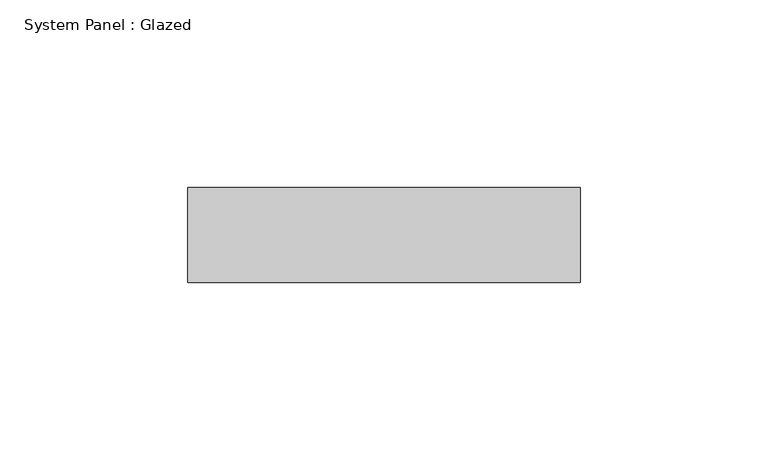
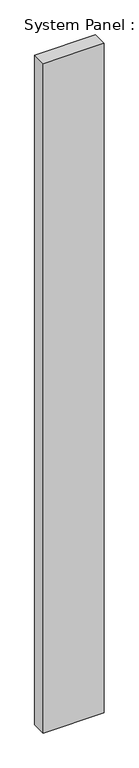
"""IFC4 building model written with IfcOpenShell, lengths in millimetres: plate geometry, System Panel : Glazed."""

import ifcopenshell
import ifcopenshell.guid

model = None  # the IFC model being written
_history = None  # IfcOwnerHistory: only IFC2X3 demands one
_inside = {}  # id of a spatial element -> (the spatial element, [elements in it])
_under = {}  # id of a project, library or spatial element -> (it, [spatial elements below it])
_declared = {}  # id of a project -> (the project, [libraries it declares])
_typed = {}  # id of a type object -> (the type object, [elements of that type])
_made_of = {}  # id of a material, layer set ... -> (it, [elements and type objects made of it])


def new_model(schema):
    """Start an empty IFC model of exactly this schema.

    Asked for "IFC4X3", IfcOpenShell would pick the latest addendum, in which some entities
    have other attributes; the version numbers below select the first issue.
    IFC2X3 requires an IfcOwnerHistory on every rooted entity: one is made here for all.
    """
    global model, _history
    if schema == "IFC4X3":
        model = ifcopenshell.file(schema_version=(4, 3, 0, 0))
    else:
        model = ifcopenshell.file(schema=schema)
    _inside.clear()
    _under.clear()
    _declared.clear()
    _typed.clear()
    _made_of.clear()
    _history = None
    if model.schema == "IFC2X3":
        org = make("IfcOrganization", Name="unknown")
        user = make(
            "IfcPersonAndOrganization",
            ThePerson=make("IfcPerson", FamilyName="unknown"),
            TheOrganization=org,
        )
        app = make(
            "IfcApplication",
            ApplicationDeveloper=org,
            Version="unknown",
            ApplicationFullName="unknown",
            ApplicationIdentifier="unknown",
        )
        _history = make(
            "IfcOwnerHistory",
            OwningUser=user,
            OwningApplication=app,
            ChangeAction="ADDED",
            CreationDate=0,
        )
    return model


def make(cls, **values):
    """One entity of the class cls with the attributes given. An attribute that is None is left unset."""
    return model.create_entity(
        cls, **{name: value for name, value in values.items() if value is not None}
    )


def rooted(cls, **values):
    """An entity with a GlobalId (a new one), such as an element, a storey or a relation."""
    return make(cls, GlobalId=ifcopenshell.guid.new(), OwnerHistory=_history, **values)


def si_unit(unit_type, name, prefix=None):
    """IfcSIUnit, for example si_unit("LENGTHUNIT", "METRE", prefix="MILLI")."""
    return make("IfcSIUnit", UnitType=unit_type, Prefix=prefix, Name=name)


def assignment(units):
    """IfcUnitAssignment: the units of a project."""
    return None if units is None else make("IfcUnitAssignment", Units=units)


def point(xyz):
    """IfcCartesianPoint."""
    return None if xyz is None else make("IfcCartesianPoint", Coordinates=xyz)


def direction(xyz):
    """IfcDirection."""
    return None if xyz is None else make("IfcDirection", DirectionRatios=xyz)


def frame(location, z_axis=None, x_axis=None):
    """IfcAxis2Placement3D, a coordinate frame: its origin and axes. An axis left out is left unset."""
    return make(
        "IfcAxis2Placement3D",
        Location=point(location),
        Axis=direction(z_axis),
        RefDirection=direction(x_axis),
    )


def origin():
    """The frame at (0, 0, 0) with its axes left unset."""
    return frame((0.0, 0.0, 0.0))


def origin_with_axes():
    """The frame at (0, 0, 0) with the z axis (0, 0, 1) and the x axis (1, 0, 0) written out."""
    return frame((0.0, 0.0, 0.0), z_axis=(0.0, 0.0, 1.0), x_axis=(1.0, 0.0, 0.0))


def place(relative_to, where):
    """IfcLocalPlacement: puts the frame where relative to a parent placement (None: the world)."""
    return make(
        "IfcLocalPlacement", PlacementRelTo=relative_to, RelativePlacement=where
    )


def context(
    kind, dimensions, precision=None, world=None, true_north=None, identifier=None
):
    """IfcGeometricRepresentationContext, for example the 3D "Model" context."""
    return make(
        "IfcGeometricRepresentationContext",
        ContextIdentifier=identifier,
        ContextType=kind,
        CoordinateSpaceDimension=dimensions,
        Precision=precision,
        WorldCoordinateSystem=world,
        TrueNorth=true_north,
    )


def project(units=None, contexts=None):
    """IfcProject with its units and contexts."""
    return rooted(
        "IfcProject",
        Name="project",
        RepresentationContexts=contexts,
        UnitsInContext=assignment(units),
    )


def spatial(cls, under=None, at=None, **own):
    """A site, building, storey or space (cls), placed at a placement, below another one or the project."""
    s = rooted(cls, ObjectPlacement=at, **own)
    if under is not None:
        _under.setdefault(under.id(), (under, []))[1].append(s)
    return s


def polyline(points):
    """IfcPolyline through the points."""
    return make("IfcPolyline", Points=[point(p) for p in points])


def outline(outer, holes=None, kind="AREA"):
    """IfcArbitraryClosedProfileDef: a profile drawn as a closed curve; with holes, ...WithVoids."""
    if holes is None:
        return make("IfcArbitraryClosedProfileDef", ProfileType=kind, OuterCurve=outer)
    return make(
        "IfcArbitraryProfileDefWithVoids",
        ProfileType=kind,
        OuterCurve=outer,
        InnerCurves=holes,
    )


def extrude(swept, where, along, depth):
    """IfcExtrudedAreaSolid: the profile swept, set in the frame where, extruded along a direction by depth."""
    return make(
        "IfcExtrudedAreaSolid",
        SweptArea=swept,
        Position=where,
        ExtrudedDirection=direction(along),
        Depth=depth,
    )


def shape(context_of_items, identifier, shape_type, items):
    """IfcShapeRepresentation: the items that make up one representation, for example the "Body"."""
    return make(
        "IfcShapeRepresentation",
        ContextOfItems=context_of_items,
        RepresentationIdentifier=identifier,
        RepresentationType=shape_type,
        Items=items,
    )


def source(mapping_origin, context_of_items, identifier, shape_type, items):
    """IfcRepresentationMap: a shape defined once, which mapped items show again and again."""
    return make(
        "IfcRepresentationMap",
        MappingOrigin=mapping_origin,
        MappedRepresentation=shape(context_of_items, identifier, shape_type, items),
    )


def transform(
    local_origin,
    x_axis=None,
    y_axis=None,
    z_axis=None,
    scale=None,
    scale2=None,
    scale3=None,
    uniform=True,
):
    """IfcCartesianTransformationOperator3D, or its non-uniform kind. x_axis, y_axis, z_axis: its Axis1, 2, 3."""
    if uniform:
        return make(
            "IfcCartesianTransformationOperator3D",
            Axis1=direction(x_axis),
            Axis2=direction(y_axis),
            LocalOrigin=point(local_origin),
            Scale=scale,
            Axis3=direction(z_axis),
        )
    return make(
        "IfcCartesianTransformationOperator3DnonUniform",
        Axis1=direction(x_axis),
        Axis2=direction(y_axis),
        LocalOrigin=point(local_origin),
        Scale=scale,
        Axis3=direction(z_axis),
        Scale2=scale2,
        Scale3=scale3,
    )


def mapped(mapping_source, mapping_target):
    """IfcMappedItem: shows the shape of a source again, moved by a transform."""
    return make(
        "IfcMappedItem", MappingSource=mapping_source, MappingTarget=mapping_target
    )


def made_of(thing, what):
    """Note that an element or type object is made of a material, layer set ...; save() writes the relation."""
    if what is not None:
        _made_of.setdefault(what.id(), (what, []))[1].append(thing)
    return thing


def element(
    cls,
    number,
    at=None,
    inside=None,
    cuts=None,
    type_object=None,
    material=None,
    context=None,
    identifier="Body",
    shape_type=None,
    held_by="IfcProductDefinitionShape",
    body=None,
    shapes=None,
    **own,
):
    """One element of the class cls, such as IfcWall. Its Tag is "e" and its number.

    at: its placement. inside: the storey or other place that contains it. cuts: it is an
    opening in that element (IfcRelVoidsElement). A single representation is given by context,
    identifier, shape_type and body (its items); several are given by shapes. held_by: the class
    of the entity that holds the representations. save() writes the other relations.
    """
    e = rooted(cls, Tag="e%d" % number, ObjectPlacement=at, **own)
    if body is not None:
        shapes = [shape(context, identifier, shape_type, body)]
    if shapes is not None:
        e.Representation = make(held_by, Representations=shapes)
    if inside is not None:
        _inside.setdefault(inside.id(), (inside, []))[1].append(e)
    if cuts is not None:
        rooted(
            "IfcRelVoidsElement", RelatingBuildingElement=cuts, RelatedOpeningElement=e
        )
    if type_object is not None:
        _typed.setdefault(type_object.id(), (type_object, []))[1].append(e)
    return made_of(e, material)


def aggregate(whole, parts):
    """IfcRelAggregates: a whole, such as a stair, and the parts it consists of."""
    return rooted("IfcRelAggregates", RelatingObject=whole, RelatedObjects=parts)


def save(model, path):
    """Write the relations noted so far, then the file.

    IfcRelAggregates (storeys below a building ...), IfcRelContainedInSpatialStructure (elements
    in a storey), IfcRelDefinesByType, IfcRelAssociatesMaterial and IfcRelDeclares: one each for
    every whole, place, type object, material and project.
    """
    for whole, parts in _under.values():
        aggregate(whole, parts)
    for where, things in _inside.values():
        rooted(
            "IfcRelContainedInSpatialStructure",
            RelatedElements=things,
            RelatingStructure=where,
        )
    for kind, things in _typed.values():
        rooted("IfcRelDefinesByType", RelatedObjects=things, RelatingType=kind)
    for what, things in _made_of.values():
        rooted("IfcRelAssociatesMaterial", RelatedObjects=things, RelatingMaterial=what)
    for by, libraries in _declared.values():
        rooted("IfcRelDeclares", RelatingContext=by, RelatedDefinitions=libraries)
    model.write(path)


def system_panel_glazed_b8bf22fe(model_context):
    return source(origin(), model_context, "Body", "SweptSolid", [
        extrude(outline(polyline([(52.3875, 19.05), (-52.3875, 19.05), (-52.3875, 44.45), (52.3875, 44.45), (52.3875, 19.05)])), origin_with_axes(), (0.0, 0.0, 1.0), 1219.2),
    ])


if __name__ == "__main__":
    model = new_model("IFC4")
    model_context = context("Model", 3, world=origin())
    ifc_project = project(units=[si_unit("LENGTHUNIT", "METRE", prefix="MILLI")], contexts=[model_context])
    site = spatial("IfcSite", under=ifc_project)
    building = spatial("IfcBuilding", under=site)
    placement = place(None, origin())
    system_panel_glazed_shape = system_panel_glazed_b8bf22fe(model_context)
    element("IfcPlate", 1, ObjectType="System Panel : Glazed", at=placement, inside=building, context=model_context, shape_type="MappedRepresentation", body=[
        mapped(system_panel_glazed_shape, transform((0.0, 0.0, 0.0), x_axis=(1.0, 0.0, 0.0), y_axis=(0.0, 1.0, 0.0), z_axis=(0.0, 0.0, 1.0))),
    ])
    save(model, "model.ifc")

# Revit data of these elements
# Element 1 (IfcPlate, "System Panel : Glazed")
#   Materials on its faces: "Glass"
# Materials
#   "Glass": class "Glass", colour RGB 0 128 192, transparency 0.75
